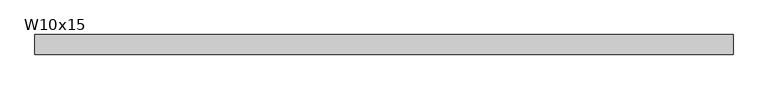
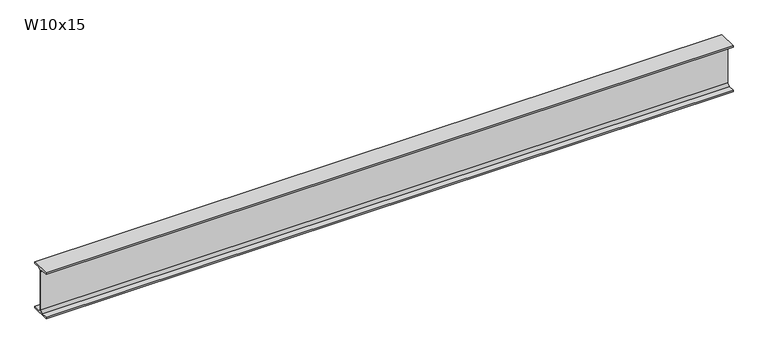
"""IFC4 building model written with IfcOpenShell, lengths in millimetres: beam geometry, RME W-Wide Flange : W10x15."""

from ifc_helpers import new_model, si_unit, point, frame, frame_2d, origin, place, context, project, spatial, polyline, circle_curve, trimmed, segment, composite_curve, outline, extrude, source, transform, mapped, element, save


def w10x15_eee40431(model_context):
    return source(origin(), model_context, "Body", "SweptSolid", [
        extrude(outline(composite_curve([segment(polyline([(50.8, -120.142), (50.8, -127.0), (-50.8, -127.0), (-50.8, -120.142), (-16.7005, -120.142)]), True, "CONTINUOUS"), segment(trimmed(circle_curve(frame_2d((-16.7005, -106.3625)), 13.7795), [point((-16.7005, -120.142))], [point((-2.921, -106.3625))], True, "CARTESIAN"), True, "CONTINUOUS"), segment(polyline([(-2.921, -106.3625), (-2.921, 106.3625)]), True, "CONTINUOUS"), segment(trimmed(circle_curve(frame_2d((-16.7005, 106.3625)), 13.7795), [point((-2.921, 106.3625))], [point((-16.7005, 120.142))], True, "CARTESIAN"), True, "CONTINUOUS"), segment(polyline([(-16.7005, 120.142), (-50.8, 120.142), (-50.8, 127.0), (50.8, 127.0), (50.8, 120.142), (16.7005, 120.142)]), True, "CONTINUOUS"), segment(trimmed(circle_curve(frame_2d((16.7005, 106.3625)), 13.7795), [point((16.7005, 120.142))], [point((2.921, 106.3625))], True, "CARTESIAN"), True, "CONTINUOUS"), segment(polyline([(2.921, 106.3625), (2.921, -106.3625)]), True, "CONTINUOUS"), segment(trimmed(circle_curve(frame_2d((16.7005, -106.3625)), 13.7795), [point((2.921, -106.3625))], [point((16.7005, -120.142))], True, "CARTESIAN"), True, "CONTINUOUS"), segment(polyline([(16.7005, -120.142), (50.8, -120.142)]), True, "CONTINUOUS")], self_intersect=False)), frame((-1809.7499994, 0.0, 0.0), z_axis=(1.0, 0.0, 0.0), x_axis=(0.0, 1.0, 0.0)), (0.0, 0.0, 1.0), 3619.4999988),
    ])


if __name__ == "__main__":
    model = new_model("IFC4")
    model_context = context("Model", 3, world=origin())
    ifc_project = project(units=[si_unit("LENGTHUNIT", "METRE", prefix="MILLI")], contexts=[model_context])
    site = spatial("IfcSite", under=ifc_project)
    building = spatial("IfcBuilding", under=site)
    placement = place(None, origin())
    w10x15_shape = w10x15_eee40431(model_context)
    element("IfcBeam", 1, ObjectType="RME W-Wide Flange : W10x15", at=placement, inside=building, context=model_context, shape_type="MappedRepresentation", body=[
        mapped(w10x15_shape, transform((0.0, 0.0, 0.0), x_axis=(1.0, 0.0, 0.0), y_axis=(0.0, 1.0, 0.0), z_axis=(0.0, 0.0, 1.0))),
    ])
    save(model, "model.ifc")

# Revit data of these elements
# Type "RME W-Wide Flange : W10x15"
#   WELD P [instance default] = ""
#   WELD LE [instance default] = ""
#   WELD D [instance default] = ""
#   TOP SECTION SIZE [instance default] = ""
#   TOP SECTION LENGTH [instance default] = ""
#   REMARKS [instance default] = ""
#   REINF TYPE [instance default] = ""
#   Nominal Size = "W24"
#   End Bearing Capacity [instance default] = ""
#   BOT SECTION SIZE [instance default] = ""
#   BOT SECTION LENGTH [instance default] = ""
#   Assembly Code = "B10"
#   W = 15
#   Start Extension Calculation [instance default] = 10' - 0"
#   Start Extension [instance default] = -0' - 0 1/2"
#   End Extension Calculation [instance default] = 10' - 0"
#   End Extension [instance default] = -0' - 0 1/2"
#   Length [instance default] = 5' - 0"
#   bf = 0' - 4"
#   d = 0' - 10"
#   k = 0' - 0 13/16"
#   k2 = 0' - 0.5425"
#   tf = 0' - 0.27"
#   tw = 0' - 0.23"
#   A = 0.030625 SF
#   Structural Material [instance default] = Metal - Steel - ASTM A992
# Element 1 (IfcBeam, "RME W-Wide Flange : W10x15")
#   Length = 11' - 11 1/2"
#   Materials on its faces: "Metal - Steel - ASTM A992"
# Materials
#   "Metal - Steel - ASTM A992": class "Metal", colour RGB 255 128 0, transparency 0
